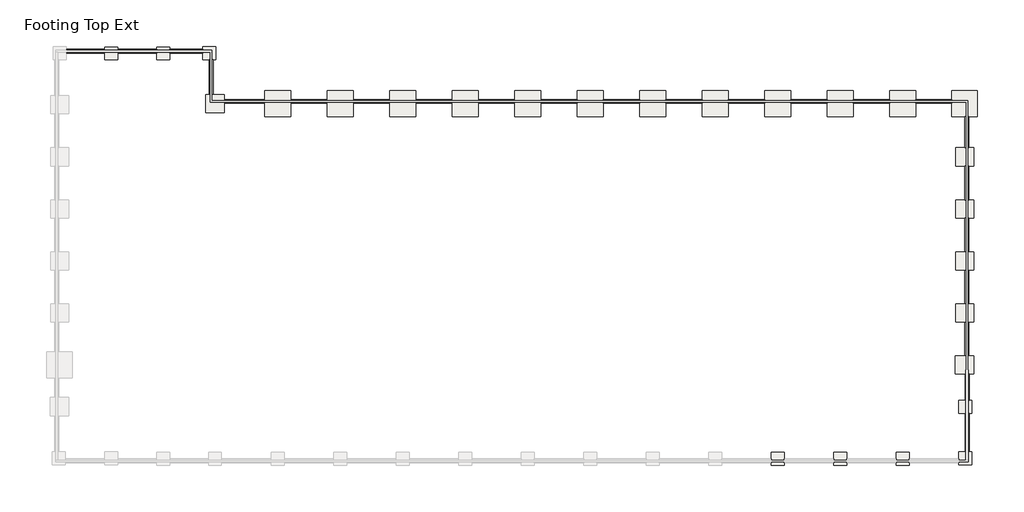
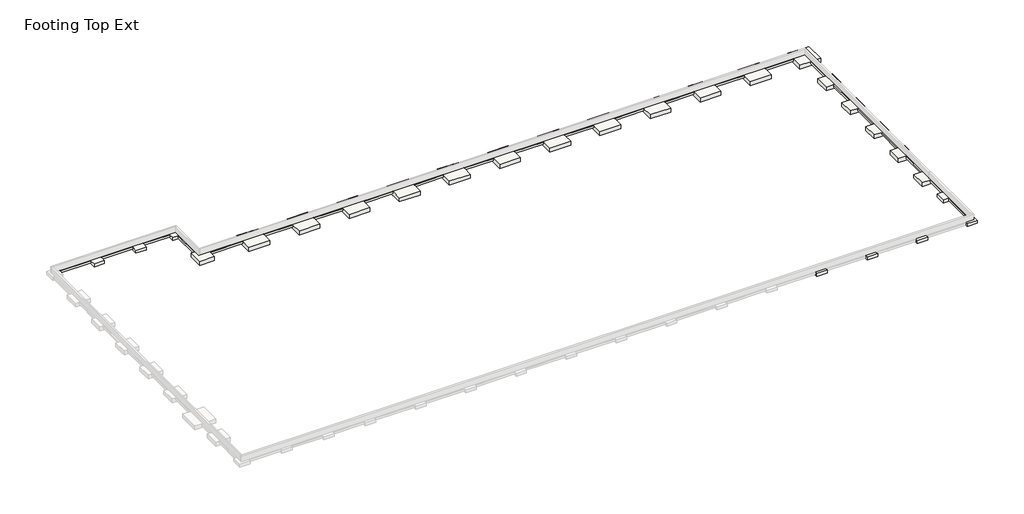
# One storey, part 2 of 2: 26 slabs, 5 footings.
"""IFC4 building model written with IfcOpenShell, lengths in millimetres."""

from ifc_helpers import new_model, si_unit, frame, origin, place, context, project, spatial, polyline, outline, extrude, faceted_brep, element, save

model = new_model("IFC4")

# Units and contexts
model_context = context("Model", 3, world=origin())
ifc_project = project(units=[si_unit("LENGTHUNIT", "METRE", prefix="MILLI")], contexts=[model_context])

# Site, building, storey
site = spatial("IfcSite", under=ifc_project)
building = spatial("IfcBuilding", under=site)
storey = spatial("IfcBuildingStorey", under=building, Name="Footing Top Ext", Elevation=-914.4)

# Footings
placement = place(None, origin())
element("IfcFooting", 1, ObjectType="Bearing Footing - 18\" x 12\"", at=placement, inside=storey, context=model_context, shape_type="SweptSolid", body=[
    extrude(outline(polyline([(305697.0398264, -530975.6413841), (305697.0398264, -530518.4413841), (310230.9398264, -530518.4413841), (310230.9398264, -530975.6413841), (305697.0398264, -530975.6413841)])), frame((0.0, 0.0, -1219.2), z_axis=(0.0, 0.0, 1.0), x_axis=(1.0, 0.0, 0.0)), (0.0, 0.0, 1.0), 304.8),
    extrude(outline(polyline([(317882.6898264, -530975.6413841), (317882.6898264, -530518.4413841), (321806.9898264, -530518.4413841), (321806.9898264, -530975.6413841), (317882.6898264, -530975.6413841)])), frame((0.0, 0.0, -1219.2), z_axis=(0.0, 0.0, 1.0), x_axis=(1.0, 0.0, 0.0)), (0.0, 0.0, 1.0), 304.8),
    extrude(outline(polyline([(316358.6898264, -530518.4413841), (316358.6898264, -530975.6413841), (311754.9398264, -530975.6413841), (311754.9398264, -530518.4413841), (316358.6898264, -530518.4413841)])), frame((0.0, 0.0, -1219.2), z_axis=(0.0, 0.0, 1.0), x_axis=(1.0, 0.0, 0.0)), (0.0, 0.0, 1.0), 304.8),
])
element("IfcFooting", 2, ObjectType="Bearing Footing - 18\" x 12\"", at=placement, inside=storey, context=model_context, shape_type="SweptSolid", body=[
    extrude(outline(polyline([(322537.2398264, -531712.2413841), (322994.4398264, -531712.2413841), (322994.4398264, -535839.7413841), (322537.2398264, -535839.7413841), (322537.2398264, -531712.2413841)])), frame((0.0, 0.0, -1219.2), z_axis=(0.0, 0.0, 1.0), x_axis=(1.0, 0.0, 0.0)), (0.0, 0.0, 1.0), 304.8),
])
element("IfcFooting", 3, ObjectType="Bearing Footing - 18\" x 12\"", at=placement, inside=storey, context=model_context, shape_type="SweptSolid", body=[
    extrude(outline(polyline([(409862.4397781, -536430.2913841), (409862.4397781, -536887.4913841), (405658.7398264, -536887.4913841), (405658.7398264, -536430.2913841), (409862.4397781, -536430.2913841)])), frame((0.0, 0.0, -1219.2), z_axis=(0.0, 0.0, 1.0), x_axis=(1.0, 0.0, 0.0)), (0.0, 0.0, 1.0), 304.8),
    extrude(outline(polyline([(402610.7398264, -536430.2913841), (402610.7398264, -536887.4913841), (398305.4398264, -536887.4913841), (398305.4398264, -536430.2913841), (402610.7398264, -536430.2913841)])), frame((0.0, 0.0, -1219.2), z_axis=(0.0, 0.0, 1.0), x_axis=(1.0, 0.0, 0.0)), (0.0, 0.0, 1.0), 304.8),
    extrude(outline(polyline([(395257.4398264, -536430.2913841), (395257.4398264, -536887.4913841), (390952.1398264, -536887.4913841), (390952.1398264, -536430.2913841), (395257.4398264, -536430.2913841)])), frame((0.0, 0.0, -1219.2), z_axis=(0.0, 0.0, 1.0), x_axis=(1.0, 0.0, 0.0)), (0.0, 0.0, 1.0), 304.8),
    extrude(outline(polyline([(387904.1398264, -536430.2913841), (387904.1398264, -536887.4913841), (383598.8398264, -536887.4913841), (383598.8398264, -536430.2913841), (387904.1398264, -536430.2913841)])), frame((0.0, 0.0, -1219.2), z_axis=(0.0, 0.0, 1.0), x_axis=(1.0, 0.0, 0.0)), (0.0, 0.0, 1.0), 304.8),
    extrude(outline(polyline([(380550.8398264, -536430.2913841), (380550.8398264, -536887.4913841), (376245.5398264, -536887.4913841), (376245.5398264, -536430.2913841), (380550.8398264, -536430.2913841)])), frame((0.0, 0.0, -1219.2), z_axis=(0.0, 0.0, 1.0), x_axis=(1.0, 0.0, 0.0)), (0.0, 0.0, 1.0), 304.8),
    extrude(outline(polyline([(373197.5398264, -536430.2913841), (373197.5398264, -536887.4913841), (368892.2398264, -536887.4913841), (368892.2398264, -536430.2913841), (373197.5398264, -536430.2913841)])), frame((0.0, 0.0, -1219.2), z_axis=(0.0, 0.0, 1.0), x_axis=(1.0, 0.0, 0.0)), (0.0, 0.0, 1.0), 304.8),
    extrude(outline(polyline([(365844.2398264, -536430.2913841), (365844.2398264, -536887.4913841), (361538.9398264, -536887.4913841), (361538.9398264, -536430.2913841), (365844.2398264, -536430.2913841)])), frame((0.0, 0.0, -1219.2), z_axis=(0.0, 0.0, 1.0), x_axis=(1.0, 0.0, 0.0)), (0.0, 0.0, 1.0), 304.8),
    extrude(outline(polyline([(358490.9398264, -536430.2913841), (358490.9398264, -536887.4913841), (354185.6398264, -536887.4913841), (354185.6398264, -536430.2913841), (358490.9398264, -536430.2913841)])), frame((0.0, 0.0, -1219.2), z_axis=(0.0, 0.0, 1.0), x_axis=(1.0, 0.0, 0.0)), (0.0, 0.0, 1.0), 304.8),
    extrude(outline(polyline([(351137.6398264, -536430.2913841), (351137.6398264, -536887.4913841), (346832.3398264, -536887.4913841), (346832.3398264, -536430.2913841), (351137.6398264, -536430.2913841)])), frame((0.0, 0.0, -1219.2), z_axis=(0.0, 0.0, 1.0), x_axis=(1.0, 0.0, 0.0)), (0.0, 0.0, 1.0), 304.8),
    extrude(outline(polyline([(343784.3398264, -536430.2913841), (343784.3398264, -536887.4913841), (339479.0398264, -536887.4913841), (339479.0398264, -536430.2913841), (343784.3398264, -536430.2913841)])), frame((0.0, 0.0, -1219.2), z_axis=(0.0, 0.0, 1.0), x_axis=(1.0, 0.0, 0.0)), (0.0, 0.0, 1.0), 304.8),
    extrude(outline(polyline([(336431.0398264, -536430.2913841), (336431.0398264, -536887.4913841), (332125.7398264, -536887.4913841), (332125.7398264, -536430.2913841), (336431.0398264, -536430.2913841)])), frame((0.0, 0.0, -1219.2), z_axis=(0.0, 0.0, 1.0), x_axis=(1.0, 0.0, 0.0)), (0.0, 0.0, 1.0), 304.8),
    extrude(outline(polyline([(329077.7398264, -536430.2913841), (329077.7398264, -536887.4913841), (324289.8398264, -536887.4913841), (324289.8398264, -536430.2913841), (329077.7398264, -536430.2913841)])), frame((0.0, 0.0, -1219.2), z_axis=(0.0, 0.0, 1.0), x_axis=(1.0, 0.0, 0.0)), (0.0, 0.0, 1.0), 304.8),
])
element("IfcFooting", 4, ObjectType="Bearing Footing - 18\" x 12\"", at=placement, inside=storey, context=model_context, shape_type="SweptSolid", body=[
    extrude(outline(polyline([(411894.4398264, -560496.7913841), (411437.2398264, -560496.7913841), (411437.2398264, -556502.6413841), (411894.4398264, -556502.6413841), (411894.4398264, -560496.7913841)])), frame((0.0, 0.0, -1219.2), z_axis=(0.0, 0.0, 1.0), x_axis=(1.0, 0.0, 0.0)), (0.0, 0.0, 1.0), 304.8),
    extrude(outline(polyline([(411437.2398264, -562630.3913841), (411894.4398264, -562630.3913841), (411894.4398264, -566599.1414082), (411437.2398264, -566599.1414082), (411437.2398264, -562630.3913841)])), frame((0.0, 0.0, -1219.2), z_axis=(0.0, 0.0, 1.0), x_axis=(1.0, 0.0, 0.0)), (0.0, 0.0, 1.0), 304.8),
    extrude(outline(polyline([(411894.4398264, -554369.0413841), (411437.2398264, -554369.0413841), (411437.2398264, -550374.8913841), (411894.4398264, -550374.8913841), (411894.4398264, -554369.0413841)])), frame((0.0, 0.0, -1219.2), z_axis=(0.0, 0.0, 1.0), x_axis=(1.0, 0.0, 0.0)), (0.0, 0.0, 1.0), 304.8),
    extrude(outline(polyline([(411894.4398264, -548241.2913841), (411437.2398264, -548241.2913841), (411437.2398264, -544247.1413841), (411894.4398264, -544247.1413841), (411894.4398264, -548241.2913841)])), frame((0.0, 0.0, -1219.2), z_axis=(0.0, 0.0, 1.0), x_axis=(1.0, 0.0, 0.0)), (0.0, 0.0, 1.0), 304.8),
    extrude(outline(polyline([(411894.4398264, -542113.5413841), (411437.2398264, -542113.5413841), (411437.2398264, -538424.1913358), (411894.4398264, -538424.1913358), (411894.4398264, -542113.5413841)])), frame((0.0, 0.0, -1219.2), z_axis=(0.0, 0.0, 1.0), x_axis=(1.0, 0.0, 0.0)), (0.0, 0.0, 1.0), 304.8),
])
element("IfcFooting", 5, ObjectType="Bearing Footing - 18\" x 12\"", at=placement, inside=storey, context=model_context, shape_type="SweptSolid", body=[
    extrude(outline(polyline([(411932.5398264, -571831.5413841), (411475.3398264, -571831.5413841), (411475.3398264, -568732.7414082), (411932.5398264, -568732.7414082), (411932.5398264, -571831.5413841)])), frame((0.0, 0.0, -1219.2), z_axis=(0.0, 0.0, 1.0), x_axis=(1.0, 0.0, 0.0)), (0.0, 0.0, 1.0), 304.8),
    extrude(outline(polyline([(411475.3398264, -573355.5413841), (411932.5398264, -573355.5413841), (411932.5398264, -577927.5413841), (411475.3398264, -577927.5413841), (411475.3398264, -573355.5413841)])), frame((0.0, 0.0, -1219.2), z_axis=(0.0, 0.0, 1.0), x_axis=(1.0, 0.0, 0.0)), (0.0, 0.0, 1.0), 304.8),
])

# Slabs
element("IfcSlab", 6, ObjectType="Footing-Rectangular : F10", at=placement, inside=storey, context=model_context, shape_type="Brep", body=[
    faceted_brep([(409862.4397781, -535376.1913358, -914.4), (409862.4397781, -536430.2913841, -914.4), (409862.4397781, -536887.4913841, -914.4), (409862.4397781, -538424.1913358, -914.4), (411437.2398264, -538424.1913358, -914.4), (411894.4398264, -538424.1913358, -914.4), (412910.4397781, -538424.1913358, -914.4), (412910.4397781, -535376.1913358, -914.4), (409862.4397781, -535376.1913358, -1524.0), (412910.4397781, -535376.1913358, -1524.0), (412910.4397781, -538424.1913358, -1524.0), (409862.4397781, -538424.1913358, -1524.0)], [[[0, 1, 2, 3, 4, 5, 6, 7]], [[8, 9, 10, 11]], [[3, 2, 1, 0, 8, 11]], [[6, 5, 4, 3, 11, 10]], [[7, 6, 10, 9]], [[0, 7, 9, 8]]]),
])
element("IfcSlab", 7, ObjectType="Footing-Rectangular : F10", at=placement, inside=storey, context=model_context, shape_type="Brep", body=[
    faceted_brep([(402610.7398264, -535382.5413358, -914.4), (402610.7398264, -536430.2913841, -914.4), (402610.7398264, -536887.4913841, -914.4), (402610.7398264, -538430.5413358, -914.4), (405658.7398264, -538430.5413358, -914.4), (405658.7398264, -536887.4913841, -914.4), (405658.7398264, -536430.2913841, -914.4), (405658.7398264, -535382.5413358, -914.4), (402610.7398264, -535382.5413358, -1524.0), (405658.7398264, -535382.5413358, -1524.0), (405658.7398264, -538430.5413358, -1524.0), (402610.7398264, -538430.5413358, -1524.0)], [[[0, 1, 2, 3, 4, 5, 6, 7]], [[8, 9, 10, 11]], [[3, 2, 1, 0, 8, 11]], [[4, 3, 11, 10]], [[7, 6, 5, 4, 10, 9]], [[0, 7, 9, 8]]]),
])
element("IfcSlab", 8, ObjectType="Footing-Rectangular : F10", at=placement, inside=storey, context=model_context, shape_type="Brep", body=[
    faceted_brep([(395257.4398264, -535382.5413358, -914.4), (395257.4398264, -536430.2913841, -914.4), (395257.4398264, -536887.4913841, -914.4), (395257.4398264, -538430.5413358, -914.4), (398305.4398264, -538430.5413358, -914.4), (398305.4398264, -536887.4913841, -914.4), (398305.4398264, -536430.2913841, -914.4), (398305.4398264, -535382.5413358, -914.4), (395257.4398264, -535382.5413358, -1524.0), (398305.4398264, -535382.5413358, -1524.0), (398305.4398264, -538430.5413358, -1524.0), (395257.4398264, -538430.5413358, -1524.0)], [[[0, 1, 2, 3, 4, 5, 6, 7]], [[8, 9, 10, 11]], [[3, 2, 1, 0, 8, 11]], [[4, 3, 11, 10]], [[7, 6, 5, 4, 10, 9]], [[0, 7, 9, 8]]]),
])
element("IfcSlab", 9, ObjectType="Footing-Rectangular : F10", at=placement, inside=storey, context=model_context, shape_type="Brep", body=[
    faceted_brep([(387904.1398264, -535382.5413358, -914.4), (387904.1398264, -536430.2913841, -914.4), (387904.1398264, -536887.4913841, -914.4), (387904.1398264, -538430.5413358, -914.4), (390952.1398264, -538430.5413358, -914.4), (390952.1398264, -536887.4913841, -914.4), (390952.1398264, -536430.2913841, -914.4), (390952.1398264, -535382.5413358, -914.4), (387904.1398264, -535382.5413358, -1524.0), (390952.1398264, -535382.5413358, -1524.0), (390952.1398264, -538430.5413358, -1524.0), (387904.1398264, -538430.5413358, -1524.0)], [[[0, 1, 2, 3, 4, 5, 6, 7]], [[8, 9, 10, 11]], [[3, 2, 1, 0, 8, 11]], [[4, 3, 11, 10]], [[7, 6, 5, 4, 10, 9]], [[0, 7, 9, 8]]]),
])
element("IfcSlab", 10, ObjectType="Footing-Rectangular : F10", at=placement, inside=storey, context=model_context, shape_type="Brep", body=[
    faceted_brep([(380550.8398264, -535382.5413358, -914.4), (380550.8398264, -536430.2913841, -914.4), (380550.8398264, -536887.4913841, -914.4), (380550.8398264, -538430.5413358, -914.4), (383598.8398264, -538430.5413358, -914.4), (383598.8398264, -536887.4913841, -914.4), (383598.8398264, -536430.2913841, -914.4), (383598.8398264, -535382.5413358, -914.4), (380550.8398264, -535382.5413358, -1524.0), (383598.8398264, -535382.5413358, -1524.0), (383598.8398264, -538430.5413358, -1524.0), (380550.8398264, -538430.5413358, -1524.0)], [[[0, 1, 2, 3, 4, 5, 6, 7]], [[8, 9, 10, 11]], [[3, 2, 1, 0, 8, 11]], [[4, 3, 11, 10]], [[7, 6, 5, 4, 10, 9]], [[0, 7, 9, 8]]]),
])
element("IfcSlab", 11, ObjectType="Footing-Rectangular : F10", at=placement, inside=storey, context=model_context, shape_type="Brep", body=[
    faceted_brep([(373197.5398264, -535382.5413358, -914.4), (373197.5398264, -536430.2913841, -914.4), (373197.5398264, -536887.4913841, -914.4), (373197.5398264, -538430.5413358, -914.4), (376245.5398264, -538430.5413358, -914.4), (376245.5398264, -536887.4913841, -914.4), (376245.5398264, -536430.2913841, -914.4), (376245.5398264, -535382.5413358, -914.4), (373197.5398264, -535382.5413358, -1524.0), (376245.5398264, -535382.5413358, -1524.0), (376245.5398264, -538430.5413358, -1524.0), (373197.5398264, -538430.5413358, -1524.0)], [[[0, 1, 2, 3, 4, 5, 6, 7]], [[8, 9, 10, 11]], [[3, 2, 1, 0, 8, 11]], [[4, 3, 11, 10]], [[7, 6, 5, 4, 10, 9]], [[0, 7, 9, 8]]]),
])
element("IfcSlab", 12, ObjectType="Footing-Rectangular : F10", at=placement, inside=storey, context=model_context, shape_type="Brep", body=[
    faceted_brep([(365844.2398264, -535382.5413358, -914.4), (365844.2398264, -536430.2913841, -914.4), (365844.2398264, -536887.4913841, -914.4), (365844.2398264, -538430.5413358, -914.4), (368892.2398264, -538430.5413358, -914.4), (368892.2398264, -536887.4913841, -914.4), (368892.2398264, -536430.2913841, -914.4), (368892.2398264, -535382.5413358, -914.4), (365844.2398264, -535382.5413358, -1524.0), (368892.2398264, -535382.5413358, -1524.0), (368892.2398264, -538430.5413358, -1524.0), (365844.2398264, -538430.5413358, -1524.0)], [[[0, 1, 2, 3, 4, 5, 6, 7]], [[8, 9, 10, 11]], [[3, 2, 1, 0, 8, 11]], [[4, 3, 11, 10]], [[7, 6, 5, 4, 10, 9]], [[0, 7, 9, 8]]]),
])
element("IfcSlab", 13, ObjectType="Footing-Rectangular : F10", at=placement, inside=storey, context=model_context, shape_type="Brep", body=[
    faceted_brep([(358490.9398264, -535382.5413358, -914.4), (358490.9398264, -536430.2913841, -914.4), (358490.9398264, -536887.4913841, -914.4), (358490.9398264, -538430.5413358, -914.4), (361538.9398264, -538430.5413358, -914.4), (361538.9398264, -536887.4913841, -914.4), (361538.9398264, -536430.2913841, -914.4), (361538.9398264, -535382.5413358, -914.4), (358490.9398264, -535382.5413358, -1524.0), (361538.9398264, -535382.5413358, -1524.0), (361538.9398264, -538430.5413358, -1524.0), (358490.9398264, -538430.5413358, -1524.0)], [[[0, 1, 2, 3, 4, 5, 6, 7]], [[8, 9, 10, 11]], [[3, 2, 1, 0, 8, 11]], [[4, 3, 11, 10]], [[7, 6, 5, 4, 10, 9]], [[0, 7, 9, 8]]]),
])
element("IfcSlab", 14, ObjectType="Footing-Rectangular : F10", at=placement, inside=storey, context=model_context, shape_type="Brep", body=[
    faceted_brep([(351137.6398264, -535382.5413358, -914.4), (351137.6398264, -536430.2913841, -914.4), (351137.6398264, -536887.4913841, -914.4), (351137.6398264, -538430.5413358, -914.4), (354185.6398264, -538430.5413358, -914.4), (354185.6398264, -536887.4913841, -914.4), (354185.6398264, -536430.2913841, -914.4), (354185.6398264, -535382.5413358, -914.4), (351137.6398264, -535382.5413358, -1524.0), (354185.6398264, -535382.5413358, -1524.0), (354185.6398264, -538430.5413358, -1524.0), (351137.6398264, -538430.5413358, -1524.0)], [[[0, 1, 2, 3, 4, 5, 6, 7]], [[8, 9, 10, 11]], [[3, 2, 1, 0, 8, 11]], [[4, 3, 11, 10]], [[7, 6, 5, 4, 10, 9]], [[0, 7, 9, 8]]]),
])
element("IfcSlab", 15, ObjectType="Footing-Rectangular : F10", at=placement, inside=storey, context=model_context, shape_type="Brep", body=[
    faceted_brep([(343784.3398264, -535382.5413358, -914.4), (343784.3398264, -536430.2913841, -914.4), (343784.3398264, -536887.4913841, -914.4), (343784.3398264, -538430.5413358, -914.4), (346832.3398264, -538430.5413358, -914.4), (346832.3398264, -536887.4913841, -914.4), (346832.3398264, -536430.2913841, -914.4), (346832.3398264, -535382.5413358, -914.4), (343784.3398264, -535382.5413358, -1524.0), (346832.3398264, -535382.5413358, -1524.0), (346832.3398264, -538430.5413358, -1524.0), (343784.3398264, -538430.5413358, -1524.0)], [[[0, 1, 2, 3, 4, 5, 6, 7]], [[8, 9, 10, 11]], [[3, 2, 1, 0, 8, 11]], [[4, 3, 11, 10]], [[7, 6, 5, 4, 10, 9]], [[0, 7, 9, 8]]]),
])
element("IfcSlab", 16, ObjectType="Footing-Rectangular : F10", at=placement, inside=storey, context=model_context, shape_type="Brep", body=[
    faceted_brep([(336431.0398264, -535382.5413358, -914.4), (336431.0398264, -536430.2913841, -914.4), (336431.0398264, -536887.4913841, -914.4), (336431.0398264, -538430.5413358, -914.4), (339479.0398264, -538430.5413358, -914.4), (339479.0398264, -536887.4913841, -914.4), (339479.0398264, -536430.2913841, -914.4), (339479.0398264, -535382.5413358, -914.4), (336431.0398264, -535382.5413358, -1524.0), (339479.0398264, -535382.5413358, -1524.0), (339479.0398264, -538430.5413358, -1524.0), (336431.0398264, -538430.5413358, -1524.0)], [[[0, 1, 2, 3, 4, 5, 6, 7]], [[8, 9, 10, 11]], [[3, 2, 1, 0, 8, 11]], [[4, 3, 11, 10]], [[7, 6, 5, 4, 10, 9]], [[0, 7, 9, 8]]]),
])
element("IfcSlab", 17, ObjectType="Footing-Rectangular : F10", at=placement, inside=storey, context=model_context, shape_type="Brep", body=[
    faceted_brep([(329077.7398264, -535382.5413358, -914.4), (329077.7398264, -536430.2913841, -914.4), (329077.7398264, -536887.4913841, -914.4), (329077.7398264, -538430.5413358, -914.4), (332125.7398264, -538430.5413358, -914.4), (332125.7398264, -536887.4913841, -914.4), (332125.7398264, -536430.2913841, -914.4), (332125.7398264, -535382.5413358, -914.4), (329077.7398264, -535382.5413358, -1524.0), (332125.7398264, -535382.5413358, -1524.0), (332125.7398264, -538430.5413358, -1524.0), (329077.7398264, -538430.5413358, -1524.0)], [[[0, 1, 2, 3, 4, 5, 6, 7]], [[8, 9, 10, 11]], [[3, 2, 1, 0, 8, 11]], [[4, 3, 11, 10]], [[7, 6, 5, 4, 10, 9]], [[0, 7, 9, 8]]]),
])
element("IfcSlab", 18, ObjectType="Footing-Rectangular : F5", at=placement, inside=storey, context=model_context, shape_type="Brep", body=[
    faceted_brep([(317882.6898264, -530245.3913841, -914.4), (316358.6898264, -530245.3913841, -914.4), (316358.6898264, -530518.4413841, -914.4), (316358.6898264, -530975.6413841, -914.4), (316358.6898264, -531769.3913841, -914.4), (317882.6898264, -531769.3913841, -914.4), (317882.6898264, -530975.6413841, -914.4), (317882.6898264, -530518.4413841, -914.4), (317882.6898264, -530245.3913841, -1371.6), (317882.6898264, -531769.3913841, -1371.6), (316358.6898264, -531769.3913841, -1371.6), (316358.6898264, -530245.3913841, -1371.6)], [[[0, 1, 2, 3, 4, 5, 6, 7]], [[8, 9, 10, 11]], [[1, 0, 8, 11]], [[4, 3, 2, 1, 11, 10]], [[5, 4, 10, 9]], [[0, 7, 6, 5, 9, 8]]]),
])
element("IfcSlab", 19, ObjectType="Footing-Rectangular : F5", at=placement, inside=storey, context=model_context, shape_type="Brep", body=[
    faceted_brep([(311754.9398264, -530245.3913841, -914.4), (310230.9398264, -530245.3913841, -914.4), (310230.9398264, -530518.4413841, -914.4), (310230.9398264, -530975.6413841, -914.4), (310230.9398264, -531769.3913841, -914.4), (311754.9398264, -531769.3913841, -914.4), (311754.9398264, -530975.6413841, -914.4), (311754.9398264, -530518.4413841, -914.4), (311754.9398264, -530245.3913841, -1371.6), (311754.9398264, -531769.3913841, -1371.6), (310230.9398264, -531769.3913841, -1371.6), (310230.9398264, -530245.3913841, -1371.6)], [[[0, 1, 2, 3, 4, 5, 6, 7]], [[8, 9, 10, 11]], [[1, 0, 8, 11]], [[4, 3, 2, 1, 11, 10]], [[5, 4, 10, 9]], [[0, 7, 6, 5, 9, 8]]]),
])
element("IfcSlab", 20, ObjectType="Footing-Rectangular : F5", at=placement, inside=storey, context=model_context, shape_type="Brep", body=[
    faceted_brep([(323330.9898264, -530188.2413841, -914.4), (321806.9898264, -530188.2413841, -914.4), (321806.9898264, -530518.4413841, -914.4), (321806.9898264, -530975.6413841, -914.4), (321806.9898264, -531712.2413841, -914.4), (322537.2398264, -531712.2413841, -914.4), (322994.4398264, -531712.2413841, -914.4), (323330.9898264, -531712.2413841, -914.4), (323330.9898264, -530188.2413841, -1371.6), (323330.9898264, -531712.2413841, -1371.6), (321806.9898264, -531712.2413841, -1371.6), (321806.9898264, -530188.2413841, -1371.6)], [[[0, 1, 2, 3, 4, 5, 6, 7]], [[8, 9, 10, 11]], [[1, 0, 8, 11]], [[4, 3, 2, 1, 11, 10]], [[7, 6, 5, 4, 10, 9]], [[0, 7, 9, 8]]]),
])
element("IfcSlab", 21, ObjectType="Footing-Rectangular : F5", at=placement, inside=storey, context=model_context, shape_type="Brep", body=[
    faceted_brep([(390190.1398264, -577978.3413841, -914.4), (388666.1398264, -577978.3413841, -914.4), (388666.1398264, -578759.3913841, -914.4), (388666.1398264, -579216.5913841, -914.4), (388666.1398264, -579502.3413841, -914.4), (390190.1398264, -579502.3413841, -914.4), (390190.1398264, -579216.5913841, -914.4), (390190.1398264, -578759.3913841, -914.4), (390190.1398264, -577978.3413841, -1371.6), (390190.1398264, -579502.3413841, -1371.6), (388666.1398264, -579502.3413841, -1371.6), (388666.1398264, -577978.3413841, -1371.6)], [[[0, 1, 2, 3, 4, 5, 6, 7]], [[8, 9, 10, 11]], [[1, 0, 8, 11]], [[4, 3, 2, 1, 11, 10]], [[5, 4, 10, 9]], [[0, 7, 6, 5, 9, 8]]]),
])
element("IfcSlab", 22, ObjectType="Footing-Rectangular : F5", at=placement, inside=storey, context=model_context, shape_type="Brep", body=[
    faceted_brep([(397543.4398264, -577971.9913841, -914.4), (396019.4398264, -577971.9913841, -914.4), (396019.4398264, -578759.3913841, -914.4), (396019.4398264, -579216.5913841, -914.4), (396019.4398264, -579495.9913841, -914.4), (397543.4398264, -579495.9913841, -914.4), (397543.4398264, -579216.5913841, -914.4), (397543.4398264, -578759.3913841, -914.4), (397543.4398264, -577971.9913841, -1371.6), (397543.4398264, -579495.9913841, -1371.6), (396019.4398264, -579495.9913841, -1371.6), (396019.4398264, -577971.9913841, -1371.6)], [[[0, 1, 2, 3, 4, 5, 6, 7]], [[8, 9, 10, 11]], [[1, 0, 8, 11]], [[4, 3, 2, 1, 11, 10]], [[5, 4, 10, 9]], [[0, 7, 6, 5, 9, 8]]]),
])
element("IfcSlab", 23, ObjectType="Footing-Rectangular : F5", at=placement, inside=storey, context=model_context, shape_type="Brep", body=[
    faceted_brep([(404896.7398264, -577971.9913841, -914.4), (403372.7398264, -577971.9913841, -914.4), (403372.7398264, -578759.3913841, -914.4), (403372.7398264, -579216.5913841, -914.4), (403372.7398264, -579495.9913841, -914.4), (404896.7398264, -579495.9913841, -914.4), (404896.7398264, -579216.5913841, -914.4), (404896.7398264, -578759.3913841, -914.4), (404896.7398264, -577971.9913841, -1371.6), (404896.7398264, -579495.9913841, -1371.6), (403372.7398264, -579495.9913841, -1371.6), (403372.7398264, -577971.9913841, -1371.6)], [[[0, 1, 2, 3, 4, 5, 6, 7]], [[8, 9, 10, 11]], [[1, 0, 8, 11]], [[4, 3, 2, 1, 11, 10]], [[5, 4, 10, 9]], [[0, 7, 6, 5, 9, 8]]]),
])
element("IfcSlab", 24, ObjectType="Footing-Rectangular : F5", at=placement, inside=storey, context=model_context, shape_type="Brep", body=[
    faceted_brep([(412218.2898264, -571831.5413841, -914.4), (411932.5398264, -571831.5413841, -914.4), (411475.3398264, -571831.5413841, -914.4), (410694.2898264, -571831.5413841, -914.4), (410694.2898264, -573355.5413841, -914.4), (411475.3398264, -573355.5413841, -914.4), (411932.5398264, -573355.5413841, -914.4), (412218.2898264, -573355.5413841, -914.4), (412218.2898264, -571831.5413841, -1371.6), (412218.2898264, -573355.5413841, -1371.6), (410694.2898264, -573355.5413841, -1371.6), (410694.2898264, -571831.5413841, -1371.6)], [[[0, 1, 2, 3, 4, 5, 6, 7]], [[8, 9, 10, 11]], [[3, 2, 1, 0, 8, 11]], [[4, 3, 11, 10]], [[7, 6, 5, 4, 10, 9]], [[0, 7, 9, 8]]]),
])
element("IfcSlab", 25, ObjectType="Footing-Rectangular : F5", at=placement, inside=storey, context=model_context, shape_type="Brep", body=[
    faceted_brep([(412224.6398264, -577927.5413841, -914.4), (411932.5398264, -577927.5413841, -914.4), (411475.3398264, -577927.5413841, -914.4), (410700.6398264, -577927.5413841, -914.4), (410700.6398264, -578759.3913841, -914.4), (410700.6398264, -579216.5913841, -914.4), (410700.6398264, -579451.5413841, -914.4), (412224.6398264, -579451.5413841, -914.4), (412224.6398264, -577927.5413841, -1371.6), (412224.6398264, -579451.5413841, -1371.6), (410700.6398264, -579451.5413841, -1371.6), (410700.6398264, -577927.5413841, -1371.6)], [[[0, 1, 2, 3, 4, 5, 6, 7]], [[8, 9, 10, 11]], [[3, 2, 1, 0, 8, 11]], [[6, 5, 4, 3, 11, 10]], [[7, 6, 10, 9]], [[0, 7, 9, 8]]]),
])
element("IfcSlab", 26, ObjectType="Footing-Rectangular : F7", at=placement, inside=storey, context=model_context, shape_type="Brep", body=[
    faceted_brep([(410319.6398264, -566599.1414082, -914.4), (410319.6398264, -568732.7414082, -914.4), (411475.3398264, -568732.7414082, -914.4), (411932.5398264, -568732.7414082, -914.4), (412453.2398264, -568732.7414082, -914.4), (412453.2398264, -566599.1414082, -914.4), (411894.4398264, -566599.1414082, -914.4), (411437.2398264, -566599.1414082, -914.4), (410319.6398264, -566599.1414082, -1524.0), (412453.2398264, -566599.1414082, -1524.0), (412453.2398264, -568732.7414082, -1524.0), (410319.6398264, -568732.7414082, -1524.0)], [[[0, 1, 2, 3, 4, 5, 6, 7]], [[8, 9, 10, 11]], [[1, 0, 8, 11]], [[4, 3, 2, 1, 11, 10]], [[5, 4, 10, 9]], [[0, 7, 6, 5, 9, 8]]]),
])
element("IfcSlab", 27, ObjectType="Footing-Rectangular : F7", at=placement, inside=storey, context=model_context, shape_type="Brep", body=[
    faceted_brep([(412484.9898264, -560496.7913841, -914.4), (411894.4398264, -560496.7913841, -914.4), (411437.2398264, -560496.7913841, -914.4), (410351.3898264, -560496.7913841, -914.4), (410351.3898264, -562630.3913841, -914.4), (411437.2398264, -562630.3913841, -914.4), (411894.4398264, -562630.3913841, -914.4), (412484.9898264, -562630.3913841, -914.4), (412484.9898264, -560496.7913841, -1524.0), (412484.9898264, -562630.3913841, -1524.0), (410351.3898264, -562630.3913841, -1524.0), (410351.3898264, -560496.7913841, -1524.0)], [[[0, 1, 2, 3, 4, 5, 6, 7]], [[8, 9, 10, 11]], [[3, 2, 1, 0, 8, 11]], [[4, 3, 11, 10]], [[7, 6, 5, 4, 10, 9]], [[0, 7, 9, 8]]]),
])
element("IfcSlab", 28, ObjectType="Footing-Rectangular : F7", at=placement, inside=storey, context=model_context, shape_type="Brep", body=[
    faceted_brep([(412484.9898264, -554369.0413841, -914.4), (411894.4398264, -554369.0413841, -914.4), (411437.2398264, -554369.0413841, -914.4), (410351.3898264, -554369.0413841, -914.4), (410351.3898264, -556502.6413841, -914.4), (411437.2398264, -556502.6413841, -914.4), (411894.4398264, -556502.6413841, -914.4), (412484.9898264, -556502.6413841, -914.4), (412484.9898264, -554369.0413841, -1524.0), (412484.9898264, -556502.6413841, -1524.0), (410351.3898264, -556502.6413841, -1524.0), (410351.3898264, -554369.0413841, -1524.0)], [[[0, 1, 2, 3, 4, 5, 6, 7]], [[8, 9, 10, 11]], [[3, 2, 1, 0, 8, 11]], [[4, 3, 11, 10]], [[7, 6, 5, 4, 10, 9]], [[0, 7, 9, 8]]]),
])
element("IfcSlab", 29, ObjectType="Footing-Rectangular : F7", at=placement, inside=storey, context=model_context, shape_type="Brep", body=[
    faceted_brep([(412484.9898264, -548241.2913841, -914.4), (411894.4398264, -548241.2913841, -914.4), (411437.2398264, -548241.2913841, -914.4), (410351.3898264, -548241.2913841, -914.4), (410351.3898264, -550374.8913841, -914.4), (411437.2398264, -550374.8913841, -914.4), (411894.4398264, -550374.8913841, -914.4), (412484.9898264, -550374.8913841, -914.4), (412484.9898264, -548241.2913841, -1524.0), (412484.9898264, -550374.8913841, -1524.0), (410351.3898264, -550374.8913841, -1524.0), (410351.3898264, -548241.2913841, -1524.0)], [[[0, 1, 2, 3, 4, 5, 6, 7]], [[8, 9, 10, 11]], [[3, 2, 1, 0, 8, 11]], [[4, 3, 11, 10]], [[7, 6, 5, 4, 10, 9]], [[0, 7, 9, 8]]]),
])
element("IfcSlab", 30, ObjectType="Footing-Rectangular : F7", at=placement, inside=storey, context=model_context, shape_type="Brep", body=[
    faceted_brep([(412478.6398264, -542113.5413841, -914.4), (411894.4398264, -542113.5413841, -914.4), (411437.2398264, -542113.5413841, -914.4), (410345.0398264, -542113.5413841, -914.4), (410345.0398264, -544247.1413841, -914.4), (411437.2398264, -544247.1413841, -914.4), (411894.4398264, -544247.1413841, -914.4), (412478.6398264, -544247.1413841, -914.4), (412478.6398264, -542113.5413841, -1524.0), (412478.6398264, -544247.1413841, -1524.0), (410345.0398264, -544247.1413841, -1524.0), (410345.0398264, -542113.5413841, -1524.0)], [[[0, 1, 2, 3, 4, 5, 6, 7]], [[8, 9, 10, 11]], [[3, 2, 1, 0, 8, 11]], [[4, 3, 11, 10]], [[7, 6, 5, 4, 10, 9]], [[0, 7, 9, 8]]]),
])
element("IfcSlab", 31, ObjectType="Footing-Rectangular : F7", at=placement, inside=storey, context=model_context, shape_type="Brep", body=[
    faceted_brep([(322156.2398264, -535839.7413841, -914.4), (322156.2398264, -537973.3413841, -914.4), (324289.8398264, -537973.3413841, -914.4), (324289.8398264, -536887.4913841, -914.4), (324289.8398264, -536430.2913841, -914.4), (324289.8398264, -535839.7413841, -914.4), (322994.4398264, -535839.7413841, -914.4), (322537.2398264, -535839.7413841, -914.4), (322156.2398264, -535839.7413841, -1524.0), (324289.8398264, -535839.7413841, -1524.0), (324289.8398264, -537973.3413841, -1524.0), (322156.2398264, -537973.3413841, -1524.0)], [[[0, 1, 2, 3, 4, 5, 6, 7]], [[8, 9, 10, 11]], [[1, 0, 8, 11]], [[2, 1, 11, 10]], [[5, 4, 3, 2, 10, 9]], [[0, 7, 6, 5, 9, 8]]]),
])

save(model, "model.ifc")

# Revit data of these elements
# Type "Bearing Footing - 18\" x 12\""
#   Assembly Code = "A1010110"
# Type "Footing-Rectangular : F10"
#   Assembly Code = "A1010100"
#   Width = 10' - 0"
#   Length = 10' - 0"
#   Thickness = 2' - 0"
#   Structural Material [instance default] = CONCRETE FOOTING - SEE STRUCT DWGS.
# Type "Footing-Rectangular : F5"
#   Assembly Code = "A1010100"
#   Width = 5' - 0"
#   Length = 5' - 0"
#   Thickness = 1' - 6"
#   Structural Material [instance default] = CONCRETE FOOTING - SEE STRUCT DWGS.
# Type "Footing-Rectangular : F7"
#   Assembly Code = "A1010100"
#   Width = 7' - 0"
#   Length = 7' - 0"
#   Thickness = 2' - 0"
#   Structural Material [instance default] = CONCRETE FOOTING - SEE STRUCT DWGS.
# Elements 1, 2, 3, 4, 5 (IfcFooting, "Bearing Footing - 18\" x 12\"")
#   Phase Created = Existing
#   Materials on its faces: "CONCRETE FOOTING - SEE STRUCT DWGS."
# Elements 6, 7, 8, 9, 10, 11, 12, 13, 14, 15, 16, 17 (IfcSlab, "Footing-Rectangular : F10")
#   Comments = ""
#   Structural Material = CONCRETE FOOTING - SEE STRUCT DWGS.
#   Phase Created = Existing
#   Materials on its faces: "CONCRETE FOOTING - SEE STRUCT DWGS."
# Elements 18, 19, 20, 21, 22, 23, 24, 25 (IfcSlab, "Footing-Rectangular : F5")
#   Comments = ""
#   Structural Material = CONCRETE FOOTING - SEE STRUCT DWGS.
#   Phase Created = Existing
#   Materials on its faces: "CONCRETE FOOTING - SEE STRUCT DWGS."
# Elements 26, 27, 28, 29, 30, 31 (IfcSlab, "Footing-Rectangular : F7")
#   Comments = ""
#   Structural Material = CONCRETE FOOTING - SEE STRUCT DWGS.
#   Phase Created = Existing
#   Materials on its faces: "CONCRETE FOOTING - SEE STRUCT DWGS."
# Materials
#   "CONCRETE FOOTING - SEE STRUCT DWGS.": class "Concrete", colour RGB 192 192 192, transparency 0, Description = "Cast-in-place concrete", Cost = 0
